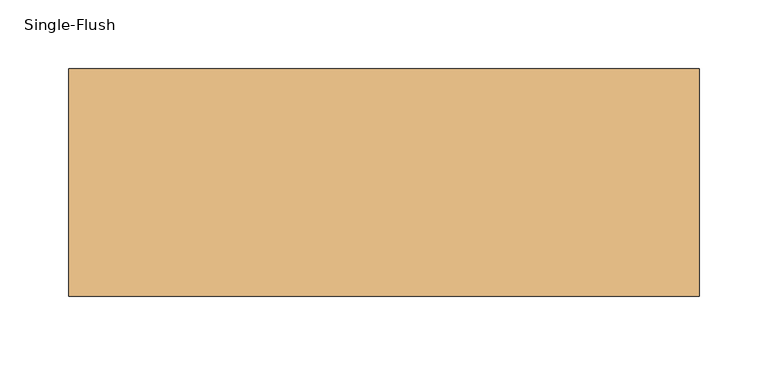
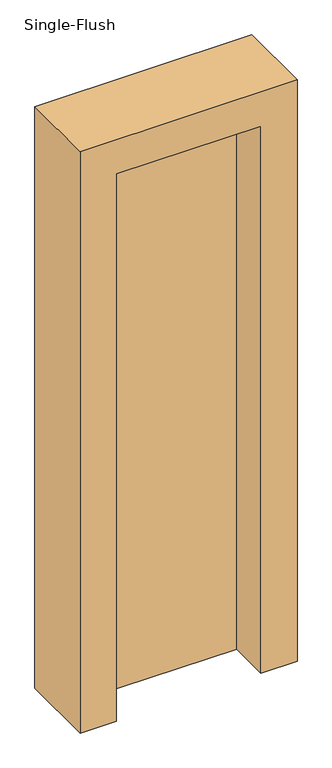
"""IFC4 building model written with IfcOpenShell, lengths in millimetres: door geometry, Single-Flush : tiny."""

import ifcopenshell
import ifcopenshell.guid

model = None  # the IFC model being written
_history = None  # IfcOwnerHistory: only IFC2X3 demands one
_inside = {}  # id of a spatial element -> (the spatial element, [elements in it])
_under = {}  # id of a project, library or spatial element -> (it, [spatial elements below it])
_declared = {}  # id of a project -> (the project, [libraries it declares])
_typed = {}  # id of a type object -> (the type object, [elements of that type])
_made_of = {}  # id of a material, layer set ... -> (it, [elements and type objects made of it])


def new_model(schema):
    """Start an empty IFC model of exactly this schema.

    Asked for "IFC4X3", IfcOpenShell would pick the latest addendum, in which some entities
    have other attributes; the version numbers below select the first issue.
    IFC2X3 requires an IfcOwnerHistory on every rooted entity: one is made here for all.
    """
    global model, _history
    if schema == "IFC4X3":
        model = ifcopenshell.file(schema_version=(4, 3, 0, 0))
    else:
        model = ifcopenshell.file(schema=schema)
    _inside.clear()
    _under.clear()
    _declared.clear()
    _typed.clear()
    _made_of.clear()
    _history = None
    if model.schema == "IFC2X3":
        org = make("IfcOrganization", Name="unknown")
        user = make(
            "IfcPersonAndOrganization",
            ThePerson=make("IfcPerson", FamilyName="unknown"),
            TheOrganization=org,
        )
        app = make(
            "IfcApplication",
            ApplicationDeveloper=org,
            Version="unknown",
            ApplicationFullName="unknown",
            ApplicationIdentifier="unknown",
        )
        _history = make(
            "IfcOwnerHistory",
            OwningUser=user,
            OwningApplication=app,
            ChangeAction="ADDED",
            CreationDate=0,
        )
    return model


def make(cls, **values):
    """One entity of the class cls with the attributes given. An attribute that is None is left unset."""
    return model.create_entity(
        cls, **{name: value for name, value in values.items() if value is not None}
    )


def rooted(cls, **values):
    """An entity with a GlobalId (a new one), such as an element, a storey or a relation."""
    return make(cls, GlobalId=ifcopenshell.guid.new(), OwnerHistory=_history, **values)


def si_unit(unit_type, name, prefix=None):
    """IfcSIUnit, for example si_unit("LENGTHUNIT", "METRE", prefix="MILLI")."""
    return make("IfcSIUnit", UnitType=unit_type, Prefix=prefix, Name=name)


def assignment(units):
    """IfcUnitAssignment: the units of a project."""
    return None if units is None else make("IfcUnitAssignment", Units=units)


def point(xyz):
    """IfcCartesianPoint."""
    return None if xyz is None else make("IfcCartesianPoint", Coordinates=xyz)


def direction(xyz):
    """IfcDirection."""
    return None if xyz is None else make("IfcDirection", DirectionRatios=xyz)


def frame(location, z_axis=None, x_axis=None):
    """IfcAxis2Placement3D, a coordinate frame: its origin and axes. An axis left out is left unset."""
    return make(
        "IfcAxis2Placement3D",
        Location=point(location),
        Axis=direction(z_axis),
        RefDirection=direction(x_axis),
    )


def origin():
    """The frame at (0, 0, 0) with its axes left unset."""
    return frame((0.0, 0.0, 0.0))


def origin_with_axes():
    """The frame at (0, 0, 0) with the z axis (0, 0, 1) and the x axis (1, 0, 0) written out."""
    return frame((0.0, 0.0, 0.0), z_axis=(0.0, 0.0, 1.0), x_axis=(1.0, 0.0, 0.0))


def place(relative_to, where):
    """IfcLocalPlacement: puts the frame where relative to a parent placement (None: the world)."""
    return make(
        "IfcLocalPlacement", PlacementRelTo=relative_to, RelativePlacement=where
    )


def context(
    kind, dimensions, precision=None, world=None, true_north=None, identifier=None
):
    """IfcGeometricRepresentationContext, for example the 3D "Model" context."""
    return make(
        "IfcGeometricRepresentationContext",
        ContextIdentifier=identifier,
        ContextType=kind,
        CoordinateSpaceDimension=dimensions,
        Precision=precision,
        WorldCoordinateSystem=world,
        TrueNorth=true_north,
    )


def project(units=None, contexts=None):
    """IfcProject with its units and contexts."""
    return rooted(
        "IfcProject",
        Name="project",
        RepresentationContexts=contexts,
        UnitsInContext=assignment(units),
    )


def spatial(cls, under=None, at=None, **own):
    """A site, building, storey or space (cls), placed at a placement, below another one or the project."""
    s = rooted(cls, ObjectPlacement=at, **own)
    if under is not None:
        _under.setdefault(under.id(), (under, []))[1].append(s)
    return s


def polyline(points):
    """IfcPolyline through the points."""
    return make("IfcPolyline", Points=[point(p) for p in points])


def outline(outer, holes=None, kind="AREA"):
    """IfcArbitraryClosedProfileDef: a profile drawn as a closed curve; with holes, ...WithVoids."""
    if holes is None:
        return make("IfcArbitraryClosedProfileDef", ProfileType=kind, OuterCurve=outer)
    return make(
        "IfcArbitraryProfileDefWithVoids",
        ProfileType=kind,
        OuterCurve=outer,
        InnerCurves=holes,
    )


def extrude(swept, where, along, depth):
    """IfcExtrudedAreaSolid: the profile swept, set in the frame where, extruded along a direction by depth."""
    return make(
        "IfcExtrudedAreaSolid",
        SweptArea=swept,
        Position=where,
        ExtrudedDirection=direction(along),
        Depth=depth,
    )


def shape(context_of_items, identifier, shape_type, items):
    """IfcShapeRepresentation: the items that make up one representation, for example the "Body"."""
    return make(
        "IfcShapeRepresentation",
        ContextOfItems=context_of_items,
        RepresentationIdentifier=identifier,
        RepresentationType=shape_type,
        Items=items,
    )


def source(mapping_origin, context_of_items, identifier, shape_type, items):
    """IfcRepresentationMap: a shape defined once, which mapped items show again and again."""
    return make(
        "IfcRepresentationMap",
        MappingOrigin=mapping_origin,
        MappedRepresentation=shape(context_of_items, identifier, shape_type, items),
    )


def transform(
    local_origin,
    x_axis=None,
    y_axis=None,
    z_axis=None,
    scale=None,
    scale2=None,
    scale3=None,
    uniform=True,
):
    """IfcCartesianTransformationOperator3D, or its non-uniform kind. x_axis, y_axis, z_axis: its Axis1, 2, 3."""
    if uniform:
        return make(
            "IfcCartesianTransformationOperator3D",
            Axis1=direction(x_axis),
            Axis2=direction(y_axis),
            LocalOrigin=point(local_origin),
            Scale=scale,
            Axis3=direction(z_axis),
        )
    return make(
        "IfcCartesianTransformationOperator3DnonUniform",
        Axis1=direction(x_axis),
        Axis2=direction(y_axis),
        LocalOrigin=point(local_origin),
        Scale=scale,
        Axis3=direction(z_axis),
        Scale2=scale2,
        Scale3=scale3,
    )


def mapped(mapping_source, mapping_target):
    """IfcMappedItem: shows the shape of a source again, moved by a transform."""
    return make(
        "IfcMappedItem", MappingSource=mapping_source, MappingTarget=mapping_target
    )


def made_of(thing, what):
    """Note that an element or type object is made of a material, layer set ...; save() writes the relation."""
    if what is not None:
        _made_of.setdefault(what.id(), (what, []))[1].append(thing)
    return thing


def element(
    cls,
    number,
    at=None,
    inside=None,
    cuts=None,
    type_object=None,
    material=None,
    context=None,
    identifier="Body",
    shape_type=None,
    held_by="IfcProductDefinitionShape",
    body=None,
    shapes=None,
    **own,
):
    """One element of the class cls, such as IfcWall. Its Tag is "e" and its number.

    at: its placement. inside: the storey or other place that contains it. cuts: it is an
    opening in that element (IfcRelVoidsElement). A single representation is given by context,
    identifier, shape_type and body (its items); several are given by shapes. held_by: the class
    of the entity that holds the representations. save() writes the other relations.
    """
    e = rooted(cls, Tag="e%d" % number, ObjectPlacement=at, **own)
    if body is not None:
        shapes = [shape(context, identifier, shape_type, body)]
    if shapes is not None:
        e.Representation = make(held_by, Representations=shapes)
    if inside is not None:
        _inside.setdefault(inside.id(), (inside, []))[1].append(e)
    if cuts is not None:
        rooted(
            "IfcRelVoidsElement", RelatingBuildingElement=cuts, RelatedOpeningElement=e
        )
    if type_object is not None:
        _typed.setdefault(type_object.id(), (type_object, []))[1].append(e)
    return made_of(e, material)


def aggregate(whole, parts):
    """IfcRelAggregates: a whole, such as a stair, and the parts it consists of."""
    return rooted("IfcRelAggregates", RelatingObject=whole, RelatedObjects=parts)


def save(model, path):
    """Write the relations noted so far, then the file.

    IfcRelAggregates (storeys below a building ...), IfcRelContainedInSpatialStructure (elements
    in a storey), IfcRelDefinesByType, IfcRelAssociatesMaterial and IfcRelDeclares: one each for
    every whole, place, type object, material and project.
    """
    for whole, parts in _under.values():
        aggregate(whole, parts)
    for where, things in _inside.values():
        rooted(
            "IfcRelContainedInSpatialStructure",
            RelatedElements=things,
            RelatingStructure=where,
        )
    for kind, things in _typed.values():
        rooted("IfcRelDefinesByType", RelatedObjects=things, RelatingType=kind)
    for what, things in _made_of.values():
        rooted("IfcRelAssociatesMaterial", RelatedObjects=things, RelatingMaterial=what)
    for by, libraries in _declared.values():
        rooted("IfcRelDeclares", RelatingContext=by, RelatedDefinitions=libraries)
    model.write(path)


def single_flush_bcd7848f(model_context):
    return source(origin(), model_context, "Body", "SweptSolid", [
        extrude(outline(polyline([(1295.4, 228.6), (1295.4, -228.6), (0.0, -228.6), (0.0, -152.4), (1219.2, -152.4), (1219.2, 152.4), (0.0, 152.4), (0.0, 228.6), (1295.4, 228.6)])), frame((0.0, -82.55, 0.0), z_axis=(0.0, 1.0, 0.0), x_axis=(0.0, 0.0, 1.0)), (0.0, 0.0, 1.0), 165.1),
        extrude(outline(polyline([(152.4, 6.35), (-152.4, 6.35), (-152.4, 57.15), (152.4, 57.15), (152.4, 6.35)])), origin_with_axes(), (0.0, 0.0, 1.0), 1219.2),
    ])


if __name__ == "__main__":
    model = new_model("IFC4")
    model_context = context("Model", 3, world=origin())
    ifc_project = project(units=[si_unit("LENGTHUNIT", "METRE", prefix="MILLI")], contexts=[model_context])
    site = spatial("IfcSite", under=ifc_project)
    building = spatial("IfcBuilding", under=site)
    placement = place(None, origin())
    single_flush_shape = single_flush_bcd7848f(model_context)
    element("IfcDoor", 1, ObjectType="Single-Flush : tiny", at=placement, inside=building, context=model_context, shape_type="MappedRepresentation", body=[
        mapped(single_flush_shape, transform((0.0, 0.0, 0.0), x_axis=(1.0, 0.0, 0.0), y_axis=(0.0, 1.0, 0.0), z_axis=(0.0, 0.0, 1.0))),
    ])
    save(model, "model.ifc")

# Revit data of these elements
# Type "Single-Flush : tiny"
#   Type Mark = "69"
#   OD_DS_Door_Material = "T.B.D."
#   OD_DS_Door_Type = "SWING"
#   OD_DS_Lockset = "PRIVACY LOCK"
#   Assembly Code = "C1020"
#   Analytic Construction = "<None>"
#   Thickness = 0' - 2"
#   RO Offset = 0' - 0 1/4"
#   Height = 4' - 0"
#   Trim Projection Ext = 0' - 1"
#   Trim Projection Int = 0' - 1"
#   Trim Width = 0' - 3"
#   Width = 1' - 0"
#   Door Material = Closet_1
#   Frame Material = Closet_1
#   Function = (empty or 0)
#   Wall Closure = (empty or 0)
# Element 1 (IfcDoor, "Single-Flush : tiny")
#   Materials on its faces: "Closet_1"
# Materials
#   "Closet_1": class "Paint", colour RGB 200 194 183, transparency 0, Cost = 0
